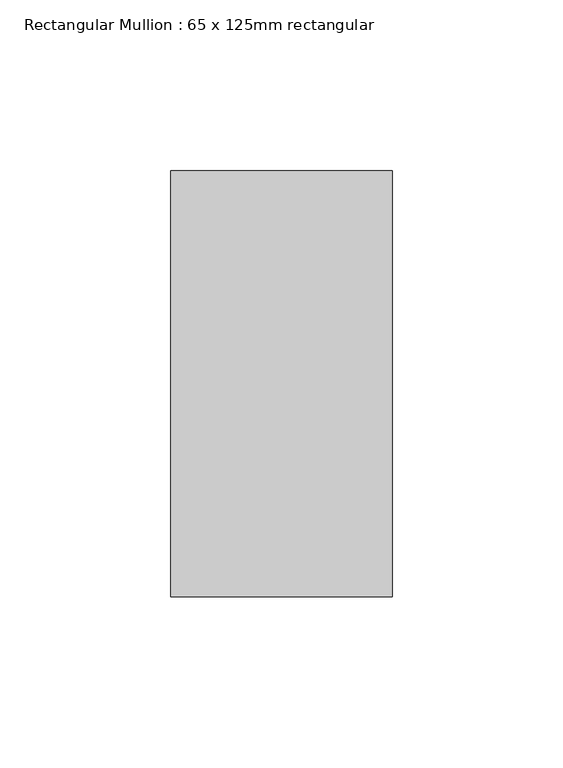
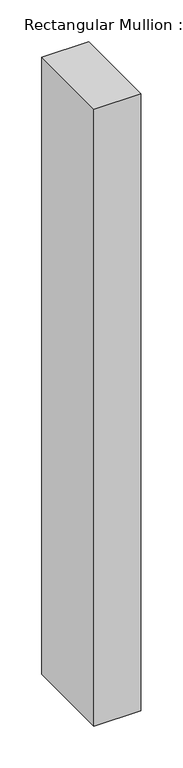
"""IFC4 building model written with IfcOpenShell, lengths in millimetres: member geometry, Rectangular Mullion : 65 x 125mm rectangular."""

from ifc_helpers import new_model, si_unit, frame, origin, place, context, project, spatial, polyline, outline, extrude, source, transform, mapped, element, save


def rectangular_mullion_65_x_125mm_rectangular_ad388592(model_context):
    return source(origin(), model_context, "Body", "SweptSolid", [
        extrude(outline(polyline([(32.5, 62.5), (32.5, -62.5), (-32.5, -62.5), (-32.5, 62.5), (32.5, 62.5)])), frame((0.0, 0.0, -902.5000003), z_axis=(0.0, 0.0, 1.0), x_axis=(1.0, 0.0, 0.0)), (0.0, 0.0, 1.0), 902.5000003),
    ])


if __name__ == "__main__":
    model = new_model("IFC4")
    model_context = context("Model", 3, world=origin())
    ifc_project = project(units=[si_unit("LENGTHUNIT", "METRE", prefix="MILLI")], contexts=[model_context])
    site = spatial("IfcSite", under=ifc_project)
    building = spatial("IfcBuilding", under=site)
    placement = place(None, origin())
    rectangular_mullion_65_x_125mm_rectangular_shape = rectangular_mullion_65_x_125mm_rectangular_ad388592(model_context)
    element("IfcMember", 1, ObjectType="Rectangular Mullion : 65 x 125mm rectangular", at=placement, inside=building, context=model_context, shape_type="MappedRepresentation", body=[
        mapped(rectangular_mullion_65_x_125mm_rectangular_shape, transform((0.0, 0.0, 0.0), x_axis=(1.0, 0.0, 0.0), y_axis=(0.0, 1.0, 0.0), z_axis=(0.0, 0.0, 1.0))),
    ])
    save(model, "model.ifc")

# Revit data of these elements
# Type "Rectangular Mullion : 65 x 125mm rectangular"
#   built-in parameter 1007304 = 0.410105 (stored number, unit not read)
#   built-in parameter 1007301 = 0.106627 (stored number, unit not read)
#   built-in parameter 1007300 = 0.106627 (stored number, unit not read)
# Element 1 (IfcMember, "Rectangular Mullion : 65 x 125mm rectangular")
#   Materials on its faces: "Aluminum"
# Materials
#   "Aluminum": class "Metal", colour RGB 244 245 246, transparency 0, Description = "Aluminum 6061", Cost = 0
